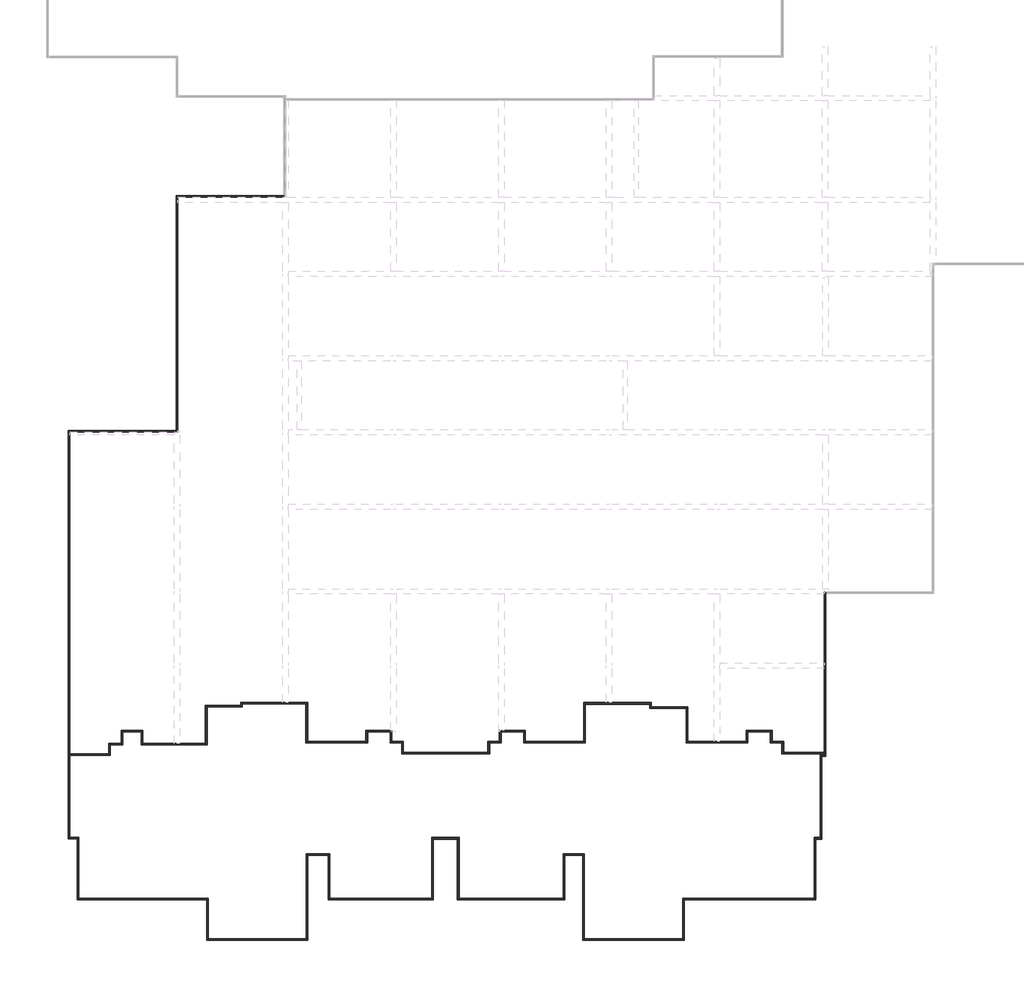
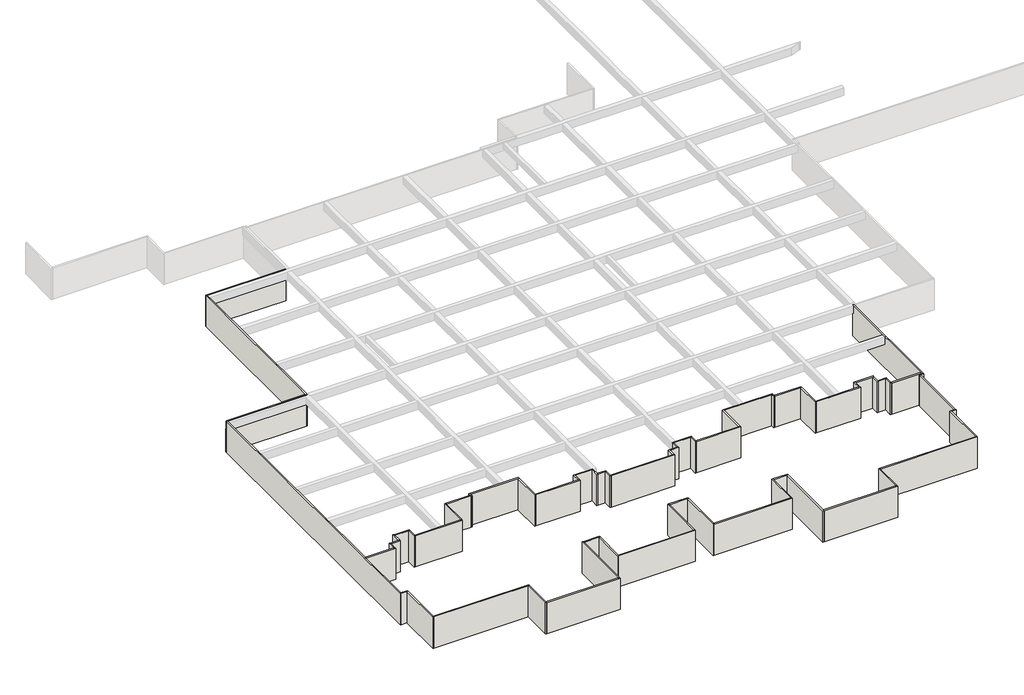
# One storey, part 1 of 14: 65 walls.
# Revit data of these elements (continued)
# Area, not placed, upper offset 0 mm, lower offset 0 mm
#   Number = "59"
#   Name = "fire_compart"
# Room, not placed, phase "新构造", upper offset 0 mm, lower offset 0 mm
#   Number = "1"
#   Name = "客餐厅"
# Room, not placed, phase "新构造", upper offset 0 mm, lower offset 0 mm
#   Number = "2"
#   Name = "阳台"
# Room, not placed, phase "新构造", upper offset 0 mm, lower offset 0 mm
#   Number = "3"
#   Name = "次卧"
# Room, not placed, phase "新构造", upper offset 0 mm, lower offset 0 mm
#   Number = "4"
#   Name = "厨房"
# Area, not placed, upper offset 0 mm, lower offset 0 mm
#   Number = "108"
#   Name = "main_building"
# Room, not placed, phase "新构造", upper offset 0 mm, lower offset 0 mm
#   Number = "5"
#   Name = "卫生间"
# Room, not placed, phase "新构造", upper offset 0 mm, lower offset 0 mm
#   Number = "6"
#   Name = "次卧"
# Room, not placed, phase "新构造", upper offset 0 mm, lower offset 0 mm
#   Number = "7"
#   Name = "主卧"
# Area, not placed, upper offset 0 mm, lower offset 0 mm
#   Number = "60"
#   Name = "fire_compart"
# Area, not placed, upper offset 0 mm, lower offset 0 mm
#   Number = "23"
#   Name = "main_building"
# Area, not placed, upper offset 0 mm, lower offset 0 mm
#   Number = "124"
#   Name = "fire_compart"
# Area, not placed, upper offset 0 mm, lower offset 0 mm
#   Number = "36"
#   Name = "main_building"
# Area, not placed, upper offset 0 mm, lower offset 0 mm
#   Number = "37"
#   Name = "main_building"
# Area, not placed, upper offset 0 mm, lower offset 0 mm
#   Number = "38"
#   Name = "main_building"
# Area, not placed, upper offset 0 mm, lower offset 0 mm
#   Number = "39"
#   Name = "main_building"
# Area, not placed, upper offset 0 mm, lower offset 0 mm
#   Number = "40"
#   Name = "main_building"
# Area, not placed, upper offset 0 mm, lower offset 0 mm
#   Number = "64"
#   Name = "fire_compart"
# Area, not placed, upper offset 0 mm, lower offset 0 mm
#   Number = "61"
#   Name = "fire_compart"
# Area, not placed, upper offset 0 mm, lower offset 0 mm
#   Number = "65"
#   Name = "main_building"
# Area, not placed, upper offset 0 mm, lower offset 0 mm
#   Number = "104"
#   Name = "main_building"
# Area, not placed, upper offset 0 mm, lower offset 0 mm
#   Number = "62"
#   Name = "fire_compart"
# Area, not placed, upper offset 0 mm, lower offset 0 mm
#   Number = "125"
#   Name = "fire_compart"
# Area, not placed, upper offset 0 mm, lower offset 0 mm
#   Number = "63"
#   Name = "fire_compart"
# Area, not placed, upper offset 0 mm, lower offset 0 mm
#   Number = "66"
#   Name = "main_building"
# Area, not placed, upper offset 0 mm, lower offset 0 mm
#   Number = "126"
#   Name = "fire_compart"
# Area, not placed, upper offset 0 mm, lower offset 0 mm
#   Number = "83"
#   Name = "fire_compart"
# Area, not placed, upper offset 0 mm, lower offset 0 mm
#   Number = "84"
#   Name = "main_building"
# Area at (-588551.144, -99713.326) mm, upper offset 0 mm, lower offset 0 mm
#   Number = "150"
#   Name = "main_building"
# Area, not placed, upper offset 0 mm, lower offset 0 mm
#   Number = "127"
#   Name = "fire_compart"
# Area, not placed, upper offset 0 mm, lower offset 0 mm
#   Number = "7"
#   Name = "fire_compart_5"
# Area, not placed, upper offset 0 mm, lower offset 0 mm
#   Number = "128"
#   Name = "fire_compart"
# Area, not placed, upper offset 0 mm, lower offset 0 mm
#   Number = "129"
#   Name = "fire_compart"
# Area at (-507749.314, -49230.18) mm, upper offset 0 mm, lower offset 0 mm
#   Number = "151"
#   Name = "main_building"
# Area, not placed, upper offset 0 mm, lower offset 0 mm
#   Number = "130"
#   Name = "fire_compart"
# Area, not placed, upper offset 0 mm, lower offset 0 mm
#   Number = "109"
#   Name = "main_building"
# Area, not placed, upper offset 0 mm, lower offset 0 mm
#   Number = "67"
#   Name = "fire_compart"
# Area, not placed, upper offset 0 mm, lower offset 0 mm
#   Number = "112"
#   Name = "main_building"
# Area, not placed, upper offset 0 mm, lower offset 0 mm
#   Number = "131"
#   Name = "fire_compart"
# Area, not placed, upper offset 0 mm, lower offset 0 mm
#   Number = "68"
#   Name = "fire_compart"
# Area at (-498982.878, -118080.719) mm, upper offset 0 mm, lower offset 0 mm
#   Number = "152"
#   Name = "main_building"
# Area, not placed, upper offset 0 mm, lower offset 0 mm
#   Number = "132"
#   Name = "fire_compart"
# Area, not placed, upper offset 0 mm, lower offset 0 mm
#   Number = "1"
#   Name = "面积"
# Area, not placed, upper offset 0 mm, lower offset 0 mm
#   Number = "2"
#   Name = "防火区域1"
# Area, not placed, upper offset 0 mm, lower offset 0 mm
#   Number = "133"
#   Name = "fire_compart"
# Area, not placed, upper offset 0 mm, lower offset 0 mm
#   Number = "144"
#   Name = "fire_compart"
# Area, not placed, upper offset 0 mm, lower offset 0 mm
#   Number = "134"
#   Name = "fire_compart"
# Area, not placed, upper offset 0 mm, lower offset 0 mm
#   Number = "25"
#   Name = "fire_compart"
# Area, not placed, upper offset 0 mm, lower offset 0 mm
#   Number = "26"
#   Name = "fire_compart"
# Area, not placed, upper offset 0 mm, lower offset 0 mm
#   Number = "27"
#   Name = "fire_compart"
# Area, not placed, upper offset 0 mm, lower offset 0 mm
#   Number = "69"
#   Name = "fire_compart"
# Area, not placed, upper offset 0 mm, lower offset 0 mm
#   Number = "105"
#   Name = "main_building"
# Area, not placed, upper offset 0 mm, lower offset 0 mm
#   Number = "113"
#   Name = "main_building"
# Area at (-565822.285, -180012.124) mm, upper offset 0 mm, lower offset 0 mm
#   Number = "153"
#   Name = "main_building"
# Area, not placed, upper offset 0 mm, lower offset 0 mm
#   Number = "135"
#   Name = "fire_compart"
# Area, not placed, upper offset 0 mm, lower offset 0 mm
#   Number = "85"
#   Name = "fire_compart"
# Area, not placed, upper offset 0 mm, lower offset 0 mm
#   Number = "86"
#   Name = "main_building"
# Area, not placed, upper offset 0 mm, lower offset 0 mm
#   Number = "87"
#   Name = "main_building"
# Area, not placed, upper offset 0 mm, lower offset 0 mm
#   Number = "136"
#   Name = "fire_compart"
# Room, not placed, phase "新构造", upper offset 0 mm, lower offset 0 mm
#   Number = "8"
#   Name = "客餐厅"
# Area, not placed, upper offset 0 mm, lower offset 0 mm
#   Number = "70"
#   Name = "main_building"
# Area at (-533396.645, -25073.922) mm, upper offset 0 mm, lower offset 0 mm
#   Number = "156"
#   Name = "fire_compart"
# Area at (-498816.194, -179494.216) mm, upper offset 0 mm, lower offset 0 mm
#   Number = "154"
#   Name = "main_building"
# Area, not placed, upper offset 0 mm, lower offset 0 mm
#   Number = "114"
#   Name = "main_building"
# Area, not placed, upper offset 0 mm, lower offset 0 mm
#   Number = "8"
#   Name = "fire_compart_6"
# Area, not placed, upper offset 0 mm, lower offset 0 mm
#   Number = "137"
#   Name = "fire_compart"
# Area, not placed, upper offset 0 mm, lower offset 0 mm
#   Number = "138"
#   Name = "fire_compart"
# Area, not placed, upper offset 0 mm, lower offset 0 mm
#   Number = "3"
#   Name = "fire_compart_1"
# Area, not placed, upper offset 0 mm, lower offset 0 mm
#   Number = "139"
#   Name = "fire_compart"
# Area, not placed, upper offset 0 mm, lower offset 0 mm
#   Number = "71"
#   Name = "fire_compart"
# Room, not placed, phase "新构造", upper offset 0 mm, lower offset 0 mm
#   Number = "11"
#   Name = "房间"
# Area, not placed, upper offset 0 mm, lower offset 0 mm
#   Number = "140"
#   Name = "fire_compart"
# Area at (-573011.453, -238576.41) mm, upper offset 0 mm, lower offset 0 mm
#   Number = "155"
#   Name = "main_building"
# Area, not placed, upper offset 0 mm, lower offset 0 mm
#   Number = "106"
#   Name = "main_building"
# Room, not placed, phase "新构造", upper offset 0 mm, lower offset 0 mm
#   Number = "12"
#   Name = "房间"
# Area, not placed, upper offset 0 mm, lower offset 0 mm
#   Number = "110"
#   Name = "main_building"
# Area, not placed, upper offset 0 mm, lower offset 0 mm
#   Number = "115"
#   Name = "main_building"
# Area, not placed, upper offset 0 mm, lower offset 0 mm
#   Number = "141"
#   Name = "fire_compart"
# Area, not placed, upper offset 0 mm, lower offset 0 mm
#   Number = "100"
#   Name = "main_building"
# Room, not placed, phase "新构造", upper offset 0 mm, lower offset 0 mm
#   Number = "13"
#   Name = "房间"
# Room, not placed, phase "新构造", upper offset 0 mm, lower offset 0 mm
#   Number = "14"
#   Name = "房间"
# Area, not placed, upper offset 0 mm, lower offset 0 mm
#   Number = "72"
#   Name = "main_building"
# Room, not placed, phase "新构造", upper offset 0 mm, lower offset 0 mm
#   Number = "15"
#   Name = "房间"
# Area, not placed, upper offset 0 mm, lower offset 0 mm
#   Number = "88"
#   Name = "fire_compart"
# Room, not placed, phase "新构造", upper offset 0 mm, lower offset 0 mm
#   Number = "16"
#   Name = "房间"
# Area, not placed, upper offset 0 mm, lower offset 0 mm
#   Number = "28"
#   Name = "面积"
# Area, not placed, upper offset 0 mm, lower offset 0 mm
#   Number = "73"
#   Name = "fire_compart"
# Area, not placed, upper offset 0 mm, lower offset 0 mm
#   Number = "116"
#   Name = "main_building"
# Area, not placed, upper offset 0 mm, lower offset 0 mm
#   Number = "101"
#   Name = "main_building"
# Room, not placed, phase "新构造", upper offset 0 mm, lower offset 0 mm
#   Number = "17"
#   Name = "房间"
# Area, not placed, upper offset 0 mm, lower offset 0 mm
#   Number = "30"
#   Name = "main_building"
# Area, not placed, upper offset 0 mm, lower offset 0 mm
#   Number = "143"
#   Name = "fire_compart"
# Area, not placed, upper offset 0 mm, lower offset 0 mm
#   Number = "89"
#   Name = "main_building"
# Area, not placed, upper offset 0 mm, lower offset 0 mm
#   Number = "75"
#   Name = "main_building"
# Area, not placed, upper offset 0 mm, lower offset 0 mm
#   Number = "111"
#   Name = "main_building"
# Area, not placed, upper offset 0 mm, lower offset 0 mm
#   Number = "90"
#   Name = "fire_compart"
# Area, not placed, upper offset 0 mm, lower offset 0 mm
#   Number = "76"
#   Name = "main_building"
# Area, not placed, upper offset 0 mm, lower offset 0 mm
#   Number = "145"
#   Name = "fire_compart"
# Area, not placed, upper offset 0 mm, lower offset 0 mm
#   Number = "146"
#   Name = "fire_compart"
# Area, not placed, upper offset 0 mm, lower offset 0 mm
#   Number = "147"
#   Name = "fire_compart"
# Area, not placed, upper offset 0 mm, lower offset 0 mm
#   Number = "117"
#   Name = "main_building"
# Area, not placed, upper offset 0 mm, lower offset 0 mm
#   Number = "4"
#   Name = "fire_compart_2"
# Area, not placed, upper offset 0 mm, lower offset 0 mm
#   Number = "77"
#   Name = "main_building"
# Area at (-542221.346, -155200.898) mm, upper offset 0 mm, lower offset 0 mm
#   Number = "159"
#   Name = "fire_compart"
# Area, not placed, upper offset 0 mm, lower offset 0 mm
#   Number = "78"
#   Name = "main_building"
# Area, not placed, upper offset 0 mm, lower offset 0 mm
#   Number = "79"
#   Name = "main_building"
# Area, not placed, upper offset 0 mm, lower offset 0 mm
#   Number = "29"
#   Name = "main_building"
